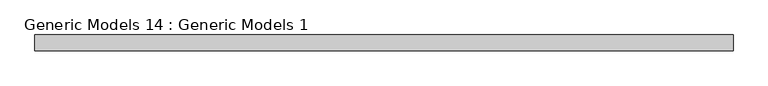
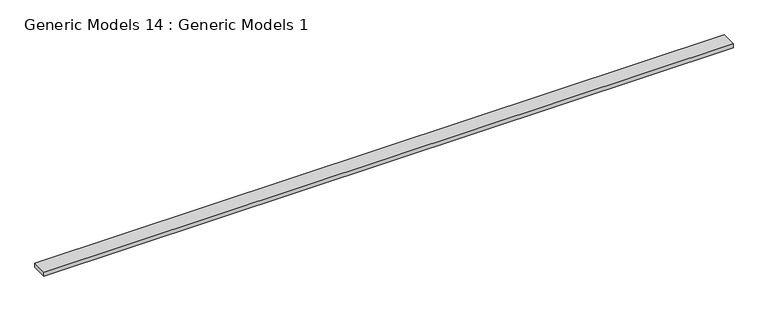
"""IFC4 building model written with IfcOpenShell, lengths in millimetres: proxy geometry, Generic Models 14 : Generic Models 1."""

from ifc_helpers import new_model, si_unit, frame, origin, place, context, project, spatial, polyline, outline, extrude, source, transform, mapped, element, save


def generic_models_14_generic_models_1_28803d39(model_context):
    return source(origin(), model_context, "Body", "SweptSolid", [
        extrude(outline(polyline([(2196.9263704, -7055.4230338), (2196.9263704, -6915.7230338), (8386.8578684, -6915.7230338), (8386.8578684, -7055.4230338), (2196.9263704, -7055.4230338)])), frame((0.0, 0.0, 126440.946), z_axis=(0.0, 0.0, 1.0), x_axis=(1.0, 0.0, 0.0)), (0.0, 0.0, 1.0), 38.1),
    ])


if __name__ == "__main__":
    model = new_model("IFC4")
    model_context = context("Model", 3, world=origin())
    ifc_project = project(units=[si_unit("LENGTHUNIT", "METRE", prefix="MILLI")], contexts=[model_context])
    site = spatial("IfcSite", under=ifc_project)
    building = spatial("IfcBuilding", under=site)
    placement = place(None, origin())
    generic_models_14_generic_models_1_shape = generic_models_14_generic_models_1_28803d39(model_context)
    element("IfcBuildingElementProxy", 1, Name="Generic Models 14 : Generic Models 1", ObjectType="Generic Models 14 : Generic Models 1", at=placement, inside=building, context=model_context, shape_type="MappedRepresentation", body=[
        mapped(generic_models_14_generic_models_1_shape, transform((0.0, 0.0, 0.0), x_axis=(1.0, 0.0, 0.0), y_axis=(0.0, 1.0, 0.0), z_axis=(0.0, 0.0, 1.0))),
    ])
    save(model, "model.ifc")

# Revit data of these elements
# Element 1 (IfcBuildingElementProxy, "Generic Models 14 : Generic Models 1")
#   Materials on its faces: "_2X BLOCKING AS REQUIRED"
# Materials
#   "_2X BLOCKING AS REQUIRED": class "Generic", colour RGB 177 130 114, transparency 0, Cost = 0
